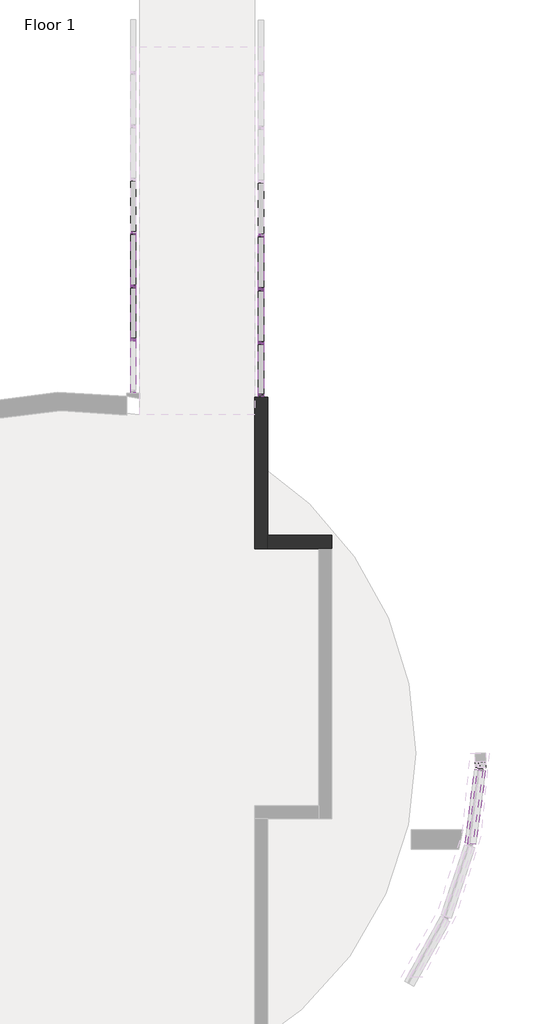
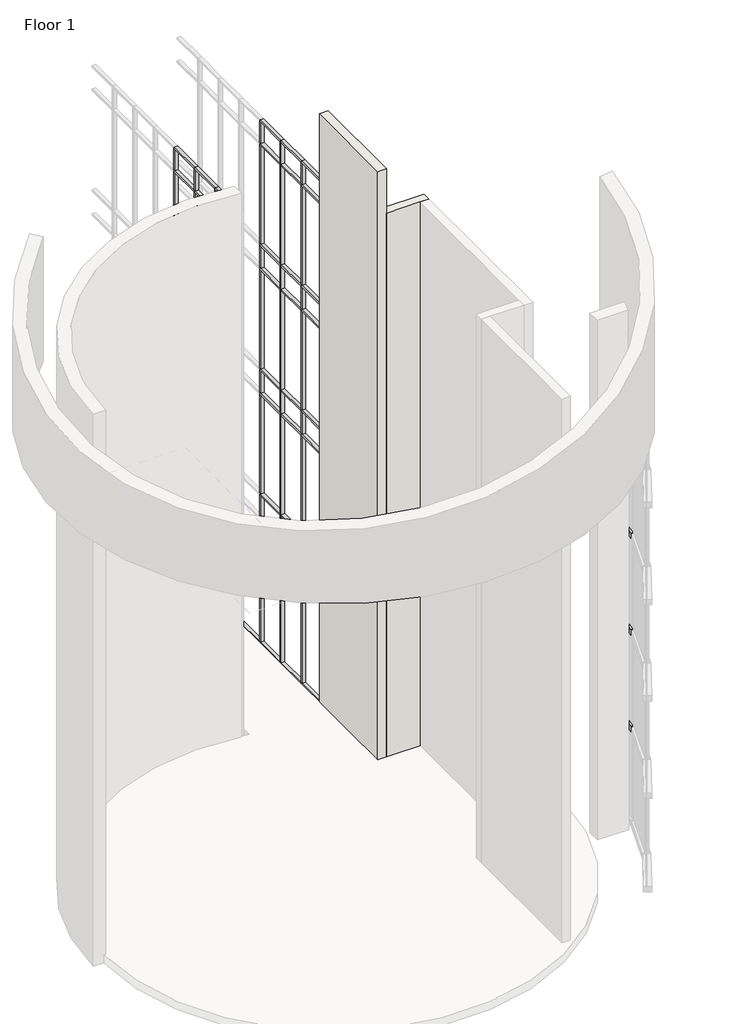
# One storey, part 7 of 11: 111 members, 2 walls.
# Revit data of these elements (continued)
# Element 112 (IfcWall, "a_Mtl panel on Mtl stud") (continued)
#   Base Constraint = Floor 1
#   Top Constraint = Roof-Bridge
#   Materials on its faces: "Default Wall", "Metal - Panel"
# Element 113 (IfcWall, "a_Mtl panel on Mtl stud")
#   Top Offset = 0' - 0"
#   Base Offset = 0' - 0"
#   wall height = 67' - 6"
#   Phase Created = New Construction
#   Base Constraint = Floor 1
#   Top Constraint = Parapet
#   Materials on its faces: "Default Wall", "Metal - Panel"
# Materials
#   "Metal - Panel": class "Unassigned", colour RGB 127 127 127, transparency 0
#   "Misc. Air Layers - Air Space": class "Miscellaneous", colour RGB 255 255 255, transparency 0
#   "Air Barrier - Air Infiltration Barrier": class "Miscellaneous", colour RGB 127 127 127, transparency 0
#   "Wood - Sheathing - plywood": class "Wood", colour RGB 212 179 113, transparency 0
#   "Metal - Stud Layer": class "Metal", colour RGB 199 199 199, transparency 0
#   "Vapor / Moisture Barriers - Vapor Retarder": class "Miscellaneous", colour RGB 127 127 127, transparency 0
#   "support-frame": class "Unassigned", colour RGB 233 233 233, transparency 0, Cost = 0
#   "Default Wall": class "Miscellaneous", colour RGB 128 128 128, transparency 0, Cost = 0
# Area at (34700.857, 51318.187) mm, upper offset 8' - 0", lower offset 0' - 0"
#   Number = "18"
#   Name = "Office Space"
# Area at (49006.684, 46244.199) mm, upper offset 8' - 0", lower offset 0' - 0"
#   Number = "19"
#   Name = "Core"
# Area at (1629.398, 48902.392) mm, upper offset 8' - 0", lower offset 0' - 0"
#   Number = "20"
#   Name = "Core"
# Area at (-5186.325, 48217.417) mm, upper offset 8' - 0", lower offset 0' - 0"
#   Number = "21"
#   Name = "Circulation"
# Area at (-13783.915, 48217.417) mm, upper offset 8' - 0", lower offset 0' - 0"
#   Number = "22"
#   Name = "Atrium"
# Area at (6186.704, 21308.019) mm, upper offset 8' - 0", lower offset 0' - 0"
#   Number = "23"
#   Name = "Office Space"
